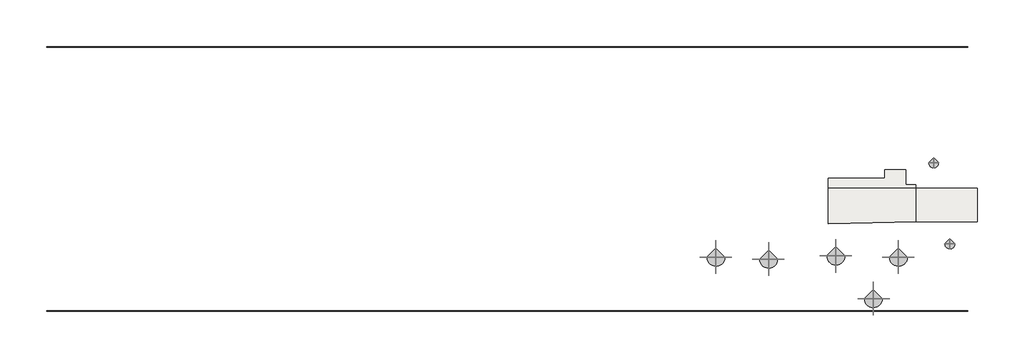
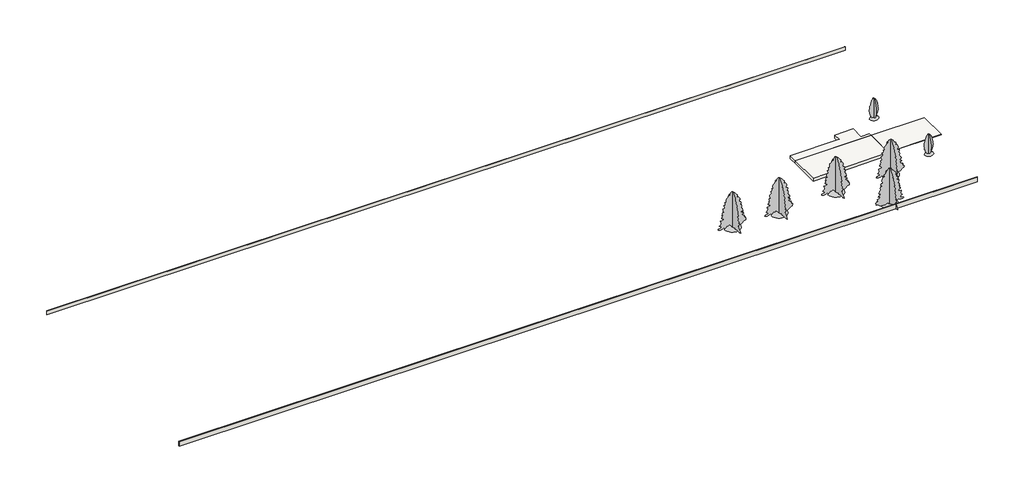
# One storey: 7 geographic elements, 3 slabs, 2 walls.
# Revit data of these elements (continued)
# Type "RPC Tree - Conifer : Chinese Juniper - 7'" (continued)
#   built-in parameter 1005198 = "{2, 15},{39, RPC-16-FUM3-UUQ0-UBF0-N000-ST1L-LVER-AU},{1, 0},{1, 0},{2, 35},{1, 8},{5, Color},{1, 0},{1, 0},{3, 0.8},{3, 0.8},{3, 0.8},{1, 8},{7, BBoxMin},{1, 0},{1, 0},{1, 0},{1, 0},{1, 0},{1, 8},{7, BBoxMax},{1, 0},{1, 0},{1, 0},{1, 0},{1, 0},{2, 11},{9, RPCTypeId},{1, 0},{1, 0},{39, RPC-16-FUM3-UUQ0-UBF0-N000-ST1L-LVER-AU},{1, 6},{14, RPCPlantHeight},{1, 0},{1, 0},{1, 7},{2, 11},{7, keyword},{1, 0},{1, 0},{96, :Geometry:RPC:Chinese Juniper:juniperus chinensis:chinese:juniper:cupressaceae:conifer:evergreen},{2, 11},{8, category},{1, 0},{1, 0},{16, :Trees [General]},{2, 11},{12, LocalizedUID},{1, 0},{1, 0},{15, Chinese Juniper},{2, 14},{6, Height},{1, 0},{1, 0},{1, 7},{1, 2},{16, Cast Reflections},{1, 0},{1, 0},{1, 0},{1, 2},{12, Cast Shadows},{1, 0},{1, 0},{1, 1},{1, 2},{9, Lock View},{1, 0},{1, 0},{1, 0},{1, 4},{5, ViewC},{1, 0},{1, 0},{1, 0},{2, 11},{20, AdvancedUIDefinition},{1, 0},{1, 0},{0, },{2, 11},{10, AssetLibID},{1, 0},{1, 0},{36, 4D3F6E72-3F99-4203-98E9-AF80B3C7A7A4},{2, 11},{10, BaseSchema},{1, 0},{1, 0},{9, RPCSchema},{2, 11},{12, ExchangeGUID},{1, 0},{1, 0},{0, },{1, 2},{6, Hidden},{1, 0},{1, 0},{1, 0},{1, 4},{11, RPCCategory},{1, 0},{1, 0},{1, 0},{2, 11},{8, RPCImage},{1, 0},{1, 0},{0, },{1, 4},{13, SchemaVersion},{1, 0},{1, 0},{1, 4},{2, 11},{12, UIDefinition},{1, 0},{1, 0},{0, },{2, 11},{6, UIName},{1, 0},{1, 0},{39, RPC-16-FUM3-UUQ0-UBF0-N000-ST1L-LVER-AU},{2, 11},{11, VersionGUID},{1, 0},{1, 0},{9, RPCSchema},{2, 11},{9, assettype},{1, 0},{1, 0},{11, RPCGeometry},{2, 11},{11, description},{1, 0},{1, 0},{0, },{2, 11},{9, localname},{1, 0},{1, 0},{3, RPC},{2, 11},{9, localtype},{1, 0},{1, 0},{3, RPC},{1, 4},{8, revision},{1, 0},{1, 0},{1, 1},{2, 11},{9, thumbnail},{1, 0},{1, 0},{0, },{1, 4},{7, version},{1, 0},{1, 0},{1, 1},{1, 2},{20, RPC_Cast Reflections},{1, 0},{1, 0},{1, 1},{1, 2},{16, RPC_Cast Shadows},{1, 0},{1, 0},{1, 1},{1, 2},{13, RPC_Lock View},{1, 0},{1, 0},{1, 0},{1, 4},{9, RPC_ViewC},{1, 0},{1, 0},{1, 0},{21, assetlibrary_base.fbx},{1, 5},"
#   built-in parameter 1005195 = "RPC-16-FUM3-UUQ0-UBF0-N000-ST1L-LVER-AU"
#   Type Comments = "Chinese Juniper"
#   Assembly Code = "G2050500"
#   Height = 213.36 cm
#   Description = (empty or 0)
#   Default Elevation = 0
# Type "aa Taban 3 cm beyaz mermer"
#   Function = 1
#   Layers, outside or top first: 3 cm "Stone" (function 1)
# Type "15mm Foundation Slab"
#   Layers, outside or top first: 3 cm "Travertine" (function 1); 30 cm "Concrete, Cast In Situ" (function 1)
# Type "aa bahçe duvarı"
#   Layers, outside or top first: 5 cm no material (function 1)
# Elements 1, 2, 3, 4, 5 (IfcGeographicElement, "RPC Tree - Conifer : Colorado Spruce - 13'")
#   Phase Created = Phase 1
# Elements 6, 7 (IfcGeographicElement, "RPC Tree - Conifer : Chinese Juniper - 7'")
#   Phase Created = Phase 1
# Element 8 (IfcSlab, "aa Taban 3 cm beyaz mermer")
#   Height Offset From Level = 0.02 cm
#   Phase Created = Phase 1
#   Materials on its faces: "Stone"
# Element 9 (IfcSlab, "15mm Foundation Slab")
#   built-in parameter 1001955 = 3.14159 (stored number, unit not read)
#   Height Offset From Level = 0 cm
#   built-in parameter 1001954 = 1
#   Phase Created = Phase 1
#   Materials on its faces: "Concrete, Cast In Situ", "Travertine"
# Element 10 (IfcSlab, "15mm Foundation Slab")
#   Height Offset From Level = 0.02 cm
#   built-in parameter 1001954 = 1
#   Phase Created = Phase 1
#   Materials on its faces: "Concrete, Cast In Situ", "Travertine"
# Element 11 (IfcWall, "aa bahçe duvarı")
#   Top Offset = 0 cm
#   Base Offset = 0 cm
#   Unconnected Height = 40 cm
#   wall height = 40 cm
#   Phase Created = Phase 1
#   Base Constraint = Bahçe
#   Materials on its faces: "Default Wall"
# Element 12 (IfcWall, "aa bahçe duvarı")
#   Top Offset = 0 cm
#   Base Offset = 0 cm
#   Unconnected Height = 50 cm
#   wall height = 50 cm
#   Phase Created = Phase 1
#   Base Constraint = Bahçe
#   Materials on its faces: "Default Wall"
# Materials
#   "Stone": class "Stone", colour RGB 120 120 120, transparency 0, Description = "Stone, rough tan", Cost = 0
#   "Travertine": class "Stone", colour RGB 120 120 120, transparency 0, Description = "Travertine, cream, matte", Cost = 0
#   "Concrete, Cast In Situ": class "Concrete", colour RGB 192 192 192, transparency 0, Description = "physical material", Cost = 0
#   "Default Wall": class "Miscellaneous", colour RGB 128 128 128, transparency 0, Cost = 0
